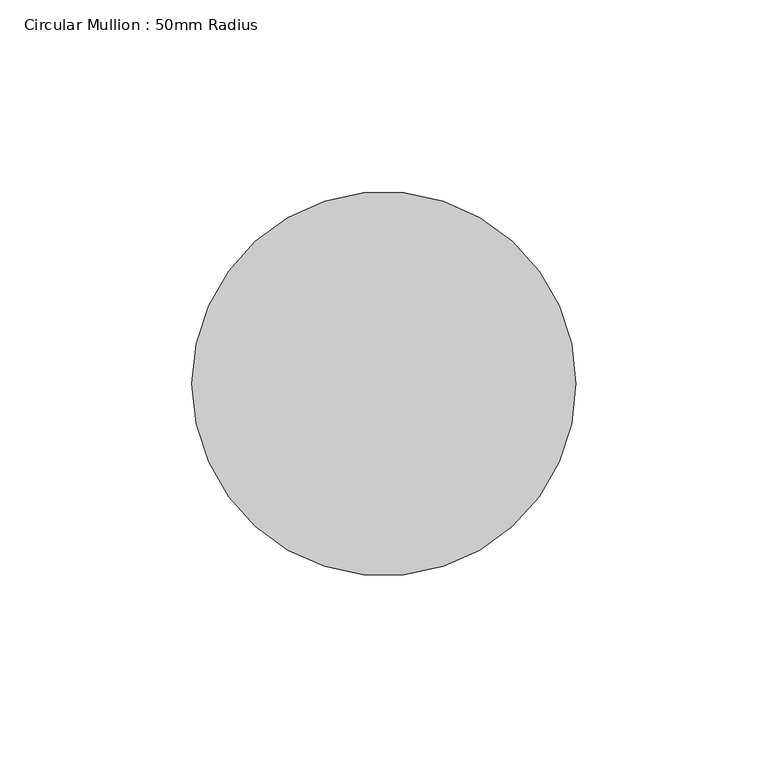
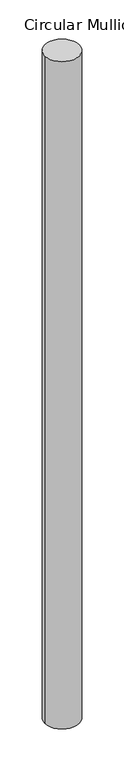
"""IFC4 building model written with IfcOpenShell, lengths in millimetres: member geometry, Circular Mullion : 50mm Radius."""

from ifc_helpers import new_model, si_unit, point, frame, frame_2d, origin, place, context, project, spatial, circle_curve, trimmed, segment, composite_curve, outline, extrude, source, transform, mapped, element, save


def circular_mullion_50mm_radius_2426858d(model_context):
    return source(origin(), model_context, "Body", "SweptSolid", [
        extrude(outline(composite_curve([segment(trimmed(circle_curve(frame_2d((-50.0, 0.0)), 50.0), [point((0.0, 0.0))], [point((-100.0, 0.0))], False, "CARTESIAN"), True, "CONTINUOUS"), segment(trimmed(circle_curve(frame_2d((-50.0, 0.0)), 50.0), [point((-100.0, 0.0))], [point((0.0, 0.0))], False, "CARTESIAN"), True, "CONTINUOUS")], self_intersect=False)), frame((0.0, 0.0, -2059.8672193), z_axis=(0.0, 0.0, 1.0), x_axis=(1.0, 0.0, 0.0)), (0.0, 0.0, 1.0), 2059.8672193),
    ])


if __name__ == "__main__":
    model = new_model("IFC4")
    model_context = context("Model", 3, world=origin())
    ifc_project = project(units=[si_unit("LENGTHUNIT", "METRE", prefix="MILLI")], contexts=[model_context])
    site = spatial("IfcSite", under=ifc_project)
    building = spatial("IfcBuilding", under=site)
    placement = place(None, origin())
    circular_mullion_50mm_radius_shape = circular_mullion_50mm_radius_2426858d(model_context)
    element("IfcMember", 1, ObjectType="Circular Mullion : 50mm Radius", at=placement, inside=building, context=model_context, shape_type="MappedRepresentation", body=[
        mapped(circular_mullion_50mm_radius_shape, transform((0.0, 0.0, 0.0), x_axis=(1.0, 0.0, 0.0), y_axis=(0.0, 1.0, 0.0), z_axis=(0.0, 0.0, 1.0))),
    ])
    save(model, "model.ifc")

# Revit data of these elements
# Type "Circular Mullion : 50mm Radius"
#   built-in parameter 1007350 = 0.164042 (stored number, unit not read)
# Element 1 (IfcMember, "Circular Mullion : 50mm Radius")
#   Materials on its faces: "Aluminium"
# Materials
#   "Aluminium": class "Metal", colour RGB 247 247 247, transparency 0, Description = "Aluminium 6061", Cost = 0
